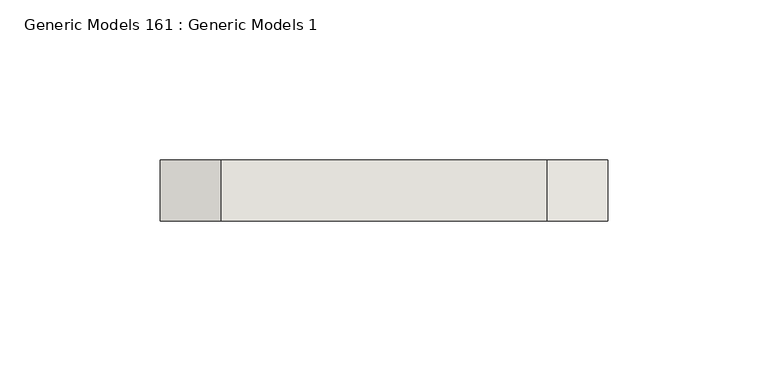
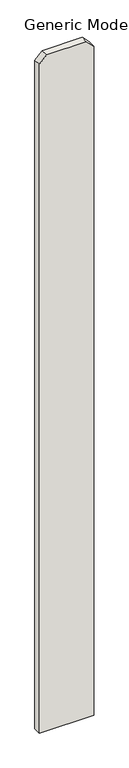
"""IFC4 building model written with IfcOpenShell, lengths in millimetres: wall geometry, Generic Models 161 : Generic Models 1."""

from ifc_helpers import new_model, si_unit, frame, origin, place, context, project, spatial, polyline, outline, extrude, source, transform, mapped, element, save


def generic_models_161_generic_models_1_31a275b3(model_context):
    return source(origin(), model_context, "Body", "SweptSolid", [
        extrude(outline(polyline([(76.2, 323518.2125), (1885.95, 323518.2125), (1905.0, 323499.1625), (1905.0, 323397.5625), (1885.95, 323378.5125), (76.2, 323378.5125), (76.2, 323518.2125)])), frame((0.0, 547.6875, 0.0), z_axis=(0.0, 1.0, 0.0), x_axis=(0.0, 0.0, 1.0)), (0.0, 0.0, 1.0), 19.05),
    ])


if __name__ == "__main__":
    model = new_model("IFC4")
    model_context = context("Model", 3, world=origin())
    ifc_project = project(units=[si_unit("LENGTHUNIT", "METRE", prefix="MILLI")], contexts=[model_context])
    site = spatial("IfcSite", under=ifc_project)
    building = spatial("IfcBuilding", under=site)
    placement = place(None, origin())
    generic_models_161_generic_models_1_shape = generic_models_161_generic_models_1_31a275b3(model_context)
    element("IfcWall", 1, ObjectType="Generic Models 161 : Generic Models 1", at=placement, inside=building, context=model_context, shape_type="MappedRepresentation", body=[
        mapped(generic_models_161_generic_models_1_shape, transform((0.0, 0.0, 0.0), x_axis=(1.0, 0.0, 0.0), y_axis=(0.0, 1.0, 0.0), z_axis=(0.0, 0.0, 1.0))),
    ])
    save(model, "model.ifc")

# Revit data of these elements
# Element 1 (IfcWall, "Generic Models 161 : Generic Models 1")
#   Materials on its faces: "VERTICAL 1X6 CEDAR PLANKS W/ CLEAR WOOD SEALER"
# Materials
#   "VERTICAL 1X6 CEDAR PLANKS W/ CLEAR WOOD SEALER": class "Wood", colour RGB 234 198 147, transparency 0, Description = "Pinus Echinata", Cost = 0
